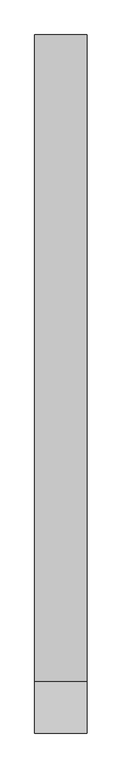
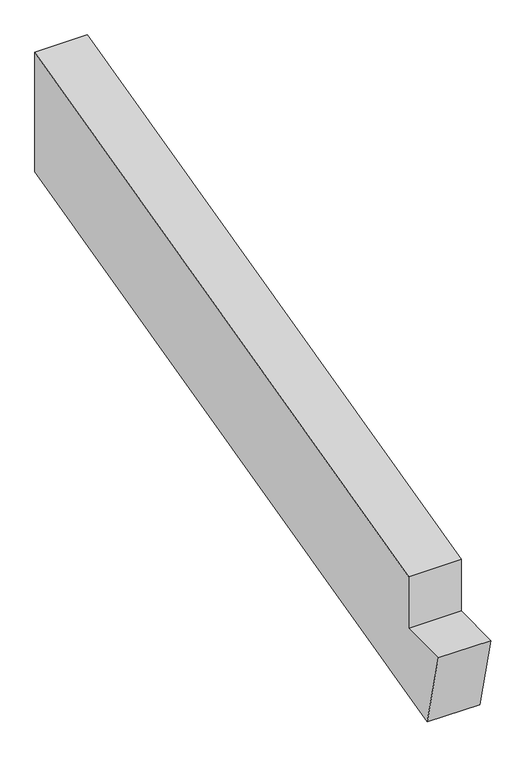
"""IFC4 building model written with IfcOpenShell, lengths in millimetres: proxy geometry, Framing024 33499 : Framing024 33499."""

from ifc_helpers import new_model, si_unit, frame, origin, place, context, project, spatial, polyline, outline, extrude, source, transform, mapped, element, save


def generic_models_9f8700c4(model_context):
    return source(origin(), model_context, "Body", "SweptSolid", [
        extrude(outline(polyline([(-5374.9745897, 42642.0307603), (-5224.4076049, 42642.0307603), (-5224.4076049, 42800.8143799), (-3344.6566162, 43270.717426), (-3344.6566162, 42903.8818003), (-5318.455674, 42411.3663805), (-5374.9745897, 42642.0307603)])), frame((13534.9, 0.0, 0.0), z_axis=(1.0, 0.0, 0.0), x_axis=(0.0, 1.0, 0.0)), (0.0, 0.0, 1.0), 152.4),
    ])


if __name__ == "__main__":
    model = new_model("IFC4")
    model_context = context("Model", 3, world=origin())
    ifc_project = project(units=[si_unit("LENGTHUNIT", "METRE", prefix="MILLI")], contexts=[model_context])
    site = spatial("IfcSite", under=ifc_project)
    building = spatial("IfcBuilding", under=site)
    placement = place(None, origin())
    generic_models_shape = generic_models_9f8700c4(model_context)
    element("IfcBuildingElementProxy", 1, Name="Framing024 33499 : Framing024 33499", ObjectType="Framing024 33499 : Framing024 33499", at=placement, inside=building, context=model_context, shape_type="MappedRepresentation", body=[
        mapped(generic_models_shape, transform((0.0, 0.0, 0.0), x_axis=(1.0, 0.0, 0.0), y_axis=(0.0, 1.0, 0.0), z_axis=(0.0, 0.0, 1.0))),
    ])
    save(model, "model.ifc")

# Revit data of these elements
# Type "Framing024 33499 : Framing024 33499"
#   NameOverride = "Framing024"
# Element 1 (IfcBuildingElementProxy, "Framing024 33499 : Framing024 33499")
#   Materials on its faces: "WOOD FRAMING (SEE STRUCT DWGS)"
# Materials
#   "WOOD FRAMING (SEE STRUCT DWGS)": class "Unassigned", colour RGB 224 188 168, transparency 0, Cost = 0
